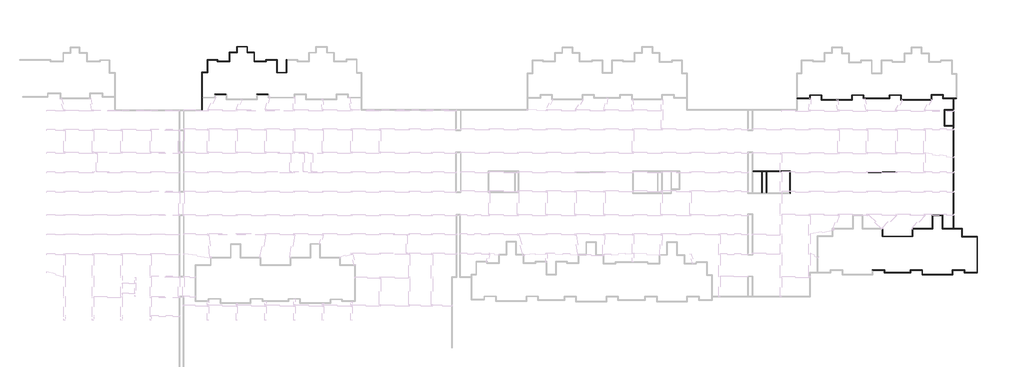
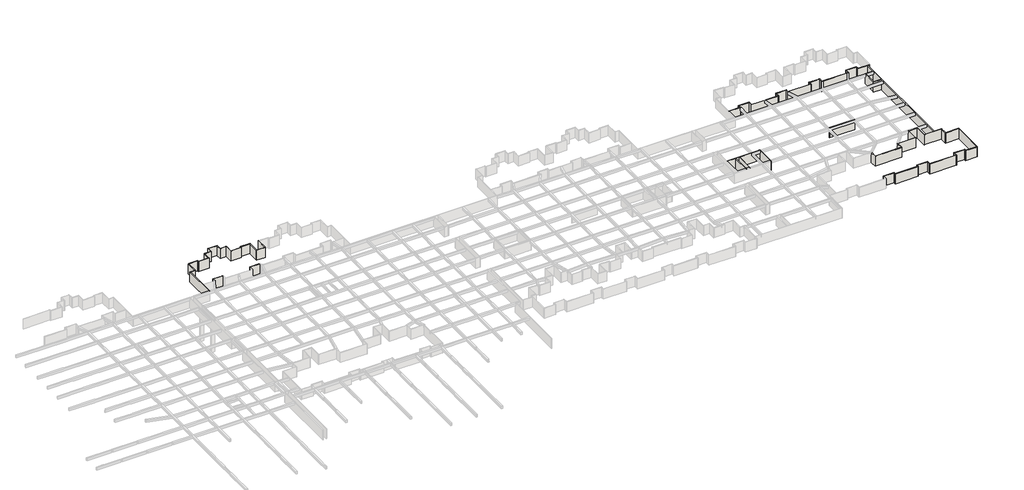
# One storey, part 7 of 16: 69 walls.
"""IFC4 building model written with IfcOpenShell, lengths in millimetres."""

from ifc_helpers import new_model, si_unit, origin, origin_with_axes, place, context, project, spatial, polyline, outline, extrude, faceted_brep, element, save

model = new_model("IFC4")

# Units and contexts
model_context = context("Model", 3, world=origin())
ifc_project = project(units=[si_unit("LENGTHUNIT", "METRE", prefix="MILLI")], contexts=[model_context])

# Site, building, storey
site = spatial("IfcSite", under=ifc_project)
building = spatial("IfcBuilding", under=site)
storey = spatial("IfcBuildingStorey", under=building, Name="户型图", Elevation=0.0)

# Walls
placement = place(None, origin())
element("IfcWall", 1, ObjectType="所有墙体", at=placement, inside=storey, context=model_context, shape_type="Brep", body=[
    faceted_brep([(261322.7517568, -132436.8999905, 0.0), (261322.7517568, -128960.8246701, 0.0), (261322.7517568, -128840.8246701, 0.0), (261322.7517568, -121956.8999905, 0.0), (261322.7517568, -121836.8999905, 0.0), (261322.7517568, -121836.8999905, 3300.0), (261322.7517568, -121956.8999905, 3300.0), (261322.7517568, -128840.8246701, 3300.0), (261322.7517568, -128960.8246701, 3300.0), (261322.7517568, -132436.8999905, 3300.0), (261202.7517568, -132436.8999905, 0.0), (261202.7517568, -132436.8999905, 3300.0), (261202.7517568, -121836.8999905, 3300.0), (261202.7517568, -121836.8999905, 0.0)], [[[0, 1, 2, 3, 4, 5, 6, 7, 8, 9]], [[10, 11, 12, 13]], [[4, 3, 2, 1, 0, 10, 13]], [[9, 8, 7, 6, 5, 12, 11]], [[0, 9, 11, 10]], [[5, 4, 13, 12]]]),
])
element("IfcWall", 2, ObjectType="所有墙体", at=placement, inside=storey, context=model_context, shape_type="Brep", body=[
    faceted_brep([(261322.7517568, -121956.8999905, 0.0), (262826.3863465, -121956.8999905, 0.0), (262826.3863465, -121956.8999905, 3300.0), (261322.7517568, -121956.8999905, 3300.0), (261322.7517568, -121836.8999905, 0.0), (261322.7517568, -121836.8999905, 3300.0), (262706.3863465, -121836.8999905, 3300.0), (262826.3863465, -121836.8999905, 3300.0), (262826.3863465, -121836.8999905, 0.0), (262706.3863465, -121836.8999905, 0.0)], [[[0, 1, 2, 3]], [[4, 5, 6, 7, 8, 9]], [[1, 0, 4, 9, 8]], [[3, 2, 7, 6, 5]], [[0, 3, 5, 4]], [[2, 1, 8, 7]]]),
])
element("IfcWall", 3, ObjectType="所有墙体", at=placement, inside=storey, context=model_context, shape_type="Brep", body=[
    faceted_brep([(262826.3863465, -121836.8999905, 0.0), (262826.3863465, -118414.1462395, 0.0), (262826.3863465, -118294.1462395, 0.0), (262826.3863465, -118294.1462395, 3300.0), (262826.3863465, -118414.1462395, 3300.0), (262826.3863465, -121836.8999905, 3300.0), (262706.3863465, -121836.8999905, 0.0), (262706.3863465, -121836.8999905, 3300.0), (262706.3863465, -118294.1462395, 3300.0), (262706.3863465, -118294.1462395, 0.0)], [[[0, 1, 2, 3, 4, 5]], [[6, 7, 8, 9]], [[2, 1, 0, 6, 9]], [[5, 4, 3, 8, 7]], [[0, 5, 7, 6]], [[3, 2, 9, 8]]]),
])
element("IfcWall", 4, ObjectType="所有墙体", at=placement, inside=storey, context=model_context, shape_type="Brep", body=[
    faceted_brep([(262826.3863465, -118414.1462395, 0.0), (265560.795916, -118414.1462395, 0.0), (265680.795916, -118414.1462395, 0.0), (265680.795916, -118414.1462395, 3300.0), (265560.795916, -118414.1462395, 3300.0), (262826.3863465, -118414.1462395, 3300.0), (262826.3863465, -118294.1462395, 0.0), (262826.3863465, -118294.1462395, 3300.0), (265680.795916, -118294.1462395, 3300.0), (265680.795916, -118294.1462395, 0.0)], [[[0, 1, 2, 3, 4, 5]], [[6, 7, 8, 9]], [[2, 1, 0, 6, 9]], [[5, 4, 3, 8, 7]], [[0, 5, 7, 6]], [[3, 2, 9, 8]]]),
])
element("IfcWall", 5, ObjectType="所有墙体", at=placement, inside=storey, context=model_context, shape_type="Brep", body=[
    faceted_brep([(265560.795916, -118414.1462395, 0.0), (265560.795916, -118816.941108, 0.0), (265560.795916, -118816.941108, 3300.0), (265560.795916, -118414.1462395, 3300.0), (265680.795916, -118414.1462395, 0.0), (265680.795916, -118414.1462395, 3300.0), (265680.795916, -118696.941108, 3300.0), (265680.795916, -118816.941108, 3300.0), (265680.795916, -118816.941108, 0.0), (265680.795916, -118696.941108, 0.0)], [[[0, 1, 2, 3]], [[4, 5, 6, 7, 8, 9]], [[1, 0, 4, 9, 8]], [[3, 2, 7, 6, 5]], [[0, 3, 5, 4]], [[2, 1, 8, 7]]]),
])
element("IfcWall", 6, ObjectType="所有墙体", at=placement, inside=storey, context=model_context, shape_type="Brep", body=[
    faceted_brep([(265680.795916, -118816.941108, 0.0), (268980.795916, -118816.941108, 0.0), (268980.795916, -118816.941108, 3300.0), (265680.795916, -118816.941108, 3300.0), (265680.795916, -118696.941108, 0.0), (265680.795916, -118696.941108, 3300.0), (268860.795916, -118696.941108, 3300.0), (268980.795916, -118696.941108, 3300.0), (268980.795916, -118696.941108, 0.0), (268860.795916, -118696.941108, 0.0)], [[[0, 1, 2, 3]], [[4, 5, 6, 7, 8, 9]], [[1, 0, 4, 9, 8]], [[3, 2, 7, 6, 5]], [[0, 3, 5, 4]], [[2, 1, 8, 7]]]),
])
element("IfcWall", 7, ObjectType="所有墙体", at=placement, inside=storey, context=model_context, shape_type="Brep", body=[
    faceted_brep([(268980.795916, -118696.941108, 0.0), (268980.795916, -116421.0126763, 0.0), (268980.795916, -116301.0126763, 0.0), (268980.795916, -116301.0126763, 3300.0), (268980.795916, -116421.0126763, 3300.0), (268980.795916, -118696.941108, 3300.0), (268860.795916, -118696.941108, 0.0), (268860.795916, -118696.941108, 3300.0), (268860.795916, -116301.0126763, 3300.0), (268860.795916, -116301.0126763, 0.0)], [[[0, 1, 2, 3, 4, 5]], [[6, 7, 8, 9]], [[2, 1, 0, 6, 9]], [[5, 4, 3, 8, 7]], [[0, 5, 7, 6]], [[3, 2, 9, 8]]]),
])
element("IfcWall", 8, ObjectType="所有墙体", at=placement, inside=storey, context=model_context, shape_type="Brep", body=[
    faceted_brep([(268980.795916, -116421.0126763, 0.0), (271083.6374023, -116421.0126763, 0.0), (271083.6374023, -116421.0126763, 3300.0), (268980.795916, -116421.0126763, 3300.0), (268980.795916, -116301.0126763, 0.0), (268980.795916, -116301.0126763, 3300.0), (270963.6374023, -116301.0126763, 3300.0), (271083.6374023, -116301.0126763, 3300.0), (271083.6374023, -116301.0126763, 0.0), (270963.6374023, -116301.0126763, 0.0)], [[[0, 1, 2, 3]], [[4, 5, 6, 7, 8, 9]], [[1, 0, 4, 9, 8]], [[3, 2, 7, 6, 5]], [[0, 3, 5, 4]], [[2, 1, 8, 7]]]),
])
element("IfcWall", 9, ObjectType="所有墙体", at=placement, inside=storey, context=model_context, shape_type="Brep", body=[
    faceted_brep([(271083.6374023, -116301.0126763, 0.0), (271083.6374023, -114773.3023088, 0.0), (271083.6374023, -114653.3023088, 0.0), (271083.6374023, -114653.3023088, 3300.0), (271083.6374023, -114773.3023088, 3300.0), (271083.6374023, -116301.0126763, 3300.0), (270963.6374023, -116301.0126763, 0.0), (270963.6374023, -116301.0126763, 3300.0), (270963.6374023, -114653.3023088, 3300.0), (270963.6374023, -114653.3023088, 0.0)], [[[0, 1, 2, 3, 4, 5]], [[6, 7, 8, 9]], [[2, 1, 0, 6, 9]], [[5, 4, 3, 8, 7]], [[0, 5, 7, 6]], [[3, 2, 9, 8]]]),
])
element("IfcWall", 10, ObjectType="所有墙体", at=placement, inside=storey, context=model_context, shape_type="Brep", body=[
    faceted_brep([(271083.6374023, -114773.3023088, 0.0), (273815.4218707, -114773.3023088, 0.0), (273935.4218707, -114773.3023088, 0.0), (273935.4218707, -114773.3023088, 3300.0), (273815.4218707, -114773.3023088, 3300.0), (271083.6374023, -114773.3023088, 3300.0), (271083.6374023, -114653.3023088, 0.0), (271083.6374023, -114653.3023088, 3300.0), (273935.4218707, -114653.3023088, 3300.0), (273935.4218707, -114653.3023088, 0.0)], [[[0, 1, 2, 3, 4, 5]], [[6, 7, 8, 9]], [[2, 1, 0, 6, 9]], [[5, 4, 3, 8, 7]], [[0, 5, 7, 6]], [[3, 2, 9, 8]]]),
])
element("IfcWall", 11, ObjectType="所有墙体", at=placement, inside=storey, context=model_context, shape_type="Brep", body=[
    faceted_brep([(273815.4218707, -114773.3023088, 0.0), (273815.4218707, -116421.0126763, 0.0), (273815.4218707, -116421.0126763, 3300.0), (273815.4218707, -114773.3023088, 3300.0), (273935.4218707, -114773.3023088, 0.0), (273935.4218707, -114773.3023088, 3300.0), (273935.4218707, -116301.0126763, 3300.0), (273935.4218707, -116421.0126763, 3300.0), (273935.4218707, -116421.0126763, 0.0), (273935.4218707, -116301.0126763, 0.0)], [[[0, 1, 2, 3]], [[4, 5, 6, 7, 8, 9]], [[1, 0, 4, 9, 8]], [[3, 2, 7, 6, 5]], [[0, 3, 5, 4]], [[2, 1, 8, 7]]]),
])
element("IfcWall", 12, ObjectType="所有墙体", at=placement, inside=storey, context=model_context, shape_type="Brep", body=[
    faceted_brep([(273935.4218707, -116421.0126763, 0.0), (275763.6122444, -116421.0126763, 0.0), (275883.6122444, -116421.0126763, 0.0), (275883.6122444, -116421.0126763, 3300.0), (275763.6122444, -116421.0126763, 3300.0), (273935.4218707, -116421.0126763, 3300.0), (273935.4218707, -116301.0126763, 0.0), (273935.4218707, -116301.0126763, 3300.0), (275883.6122444, -116301.0126763, 3300.0), (275883.6122444, -116301.0126763, 0.0)], [[[0, 1, 2, 3, 4, 5]], [[6, 7, 8, 9]], [[2, 1, 0, 6, 9]], [[5, 4, 3, 8, 7]], [[0, 5, 7, 6]], [[3, 2, 9, 8]]]),
])
element("IfcWall", 13, ObjectType="所有墙体", at=placement, inside=storey, context=model_context, shape_type="Brep", body=[
    faceted_brep([(275763.6122444, -116421.0126763, 0.0), (275763.6122444, -118816.941108, 0.0), (275763.6122444, -118816.941108, 3300.0), (275763.6122444, -116421.0126763, 3300.0), (275883.6122444, -116421.0126763, 0.0), (275883.6122444, -116421.0126763, 3300.0), (275883.6122444, -118696.941108, 3300.0), (275883.6122444, -118816.941108, 3300.0), (275883.6122444, -118816.941108, 0.0), (275883.6122444, -118696.941108, 0.0)], [[[0, 1, 2, 3]], [[4, 5, 6, 7, 8, 9]], [[1, 0, 4, 9, 8]], [[3, 2, 7, 6, 5]], [[0, 3, 5, 4]], [[2, 1, 8, 7]]]),
])
element("IfcWall", 14, ObjectType="所有墙体", at=placement, inside=storey, context=model_context, shape_type="Brep", body=[
    faceted_brep([(275883.6122444, -118816.941108, 0.0), (279180.1877082, -118816.941108, 0.0), (279180.1877082, -118816.941108, 3300.0), (275883.6122444, -118816.941108, 3300.0), (275883.6122444, -118696.941108, 0.0), (275883.6122444, -118696.941108, 3300.0), (279060.1877082, -118696.941108, 3300.0), (279180.1877082, -118696.941108, 3300.0), (279180.1877082, -118696.941108, 0.0), (279060.1877082, -118696.941108, 0.0)], [[[0, 1, 2, 3]], [[4, 5, 6, 7, 8, 9]], [[1, 0, 4, 9, 8]], [[3, 2, 7, 6, 5]], [[0, 3, 5, 4]], [[2, 1, 8, 7]]]),
])
element("IfcWall", 15, ObjectType="所有墙体", at=placement, inside=storey, context=model_context, shape_type="Brep", body=[
    faceted_brep([(279180.1877082, -118696.941108, 0.0), (279180.1877082, -118416.941108, 0.0), (279180.1877082, -118296.941108, 0.0), (279180.1877082, -118296.941108, 3300.0), (279180.1877082, -118416.941108, 3300.0), (279180.1877082, -118696.941108, 3300.0), (279060.1877082, -118696.941108, 0.0), (279060.1877082, -118696.941108, 3300.0), (279060.1877082, -118296.941108, 3300.0), (279060.1877082, -118296.941108, 0.0)], [[[0, 1, 2, 3, 4, 5]], [[6, 7, 8, 9]], [[2, 1, 0, 6, 9]], [[5, 4, 3, 8, 7]], [[0, 5, 7, 6]], [[3, 2, 9, 8]]]),
])
element("IfcWall", 16, ObjectType="所有墙体", at=placement, inside=storey, context=model_context, shape_type="Brep", body=[
    faceted_brep([(279180.1877082, -118416.941108, 0.0), (282060.1877082, -118416.941108, 0.0), (282180.1877082, -118416.941108, 0.0), (282180.1877082, -118416.941108, 3300.0), (282060.1877082, -118416.941108, 3300.0), (279180.1877082, -118416.941108, 3300.0), (279180.1877082, -118296.941108, 0.0), (279180.1877082, -118296.941108, 3300.0), (282180.1877082, -118296.941108, 3300.0), (282180.1877082, -118296.941108, 0.0)], [[[0, 1, 2, 3, 4, 5]], [[6, 7, 8, 9]], [[2, 1, 0, 6, 9]], [[5, 4, 3, 8, 7]], [[0, 5, 7, 6]], [[3, 2, 9, 8]]]),
])
element("IfcWall", 17, ObjectType="所有墙体", at=placement, inside=storey, context=model_context, shape_type="Brep", body=[
    faceted_brep([(282060.1877082, -118416.941108, 0.0), (282060.1877082, -122016.941108, 0.0), (282060.1877082, -122016.941108, 3300.0), (282060.1877082, -118416.941108, 3300.0), (282180.1877082, -118416.941108, 0.0), (282180.1877082, -118416.941108, 3300.0), (282180.1877082, -121896.941108, 3300.0), (282180.1877082, -122016.941108, 3300.0), (282180.1877082, -122016.941108, 0.0), (282180.1877082, -121896.941108, 0.0)], [[[0, 1, 2, 3]], [[4, 5, 6, 7, 8, 9]], [[1, 0, 4, 9, 8]], [[3, 2, 7, 6, 5]], [[0, 3, 5, 4]], [[2, 1, 8, 7]]]),
])
element("IfcWall", 18, ObjectType="所有墙体", at=placement, inside=storey, context=model_context, shape_type="Brep", body=[
    faceted_brep([(282180.1877082, -122016.941108, 0.0), (284876.4528769, -122016.941108, 0.0), (284876.4528769, -122016.941108, 3300.0), (282180.1877082, -122016.941108, 3300.0), (282180.1877082, -121896.941108, 0.0), (282180.1877082, -121896.941108, 3300.0), (284756.4528769, -121896.941108, 3300.0), (284876.4528769, -121896.941108, 3300.0), (284876.4528769, -121896.941108, 0.0), (284756.4528769, -121896.941108, 0.0)], [[[0, 1, 2, 3]], [[4, 5, 6, 7, 8, 9]], [[1, 0, 4, 9, 8]], [[3, 2, 7, 6, 5]], [[0, 3, 5, 4]], [[2, 1, 8, 7]]]),
])
element("IfcWall", 19, ObjectType="所有墙体", at=placement, inside=storey, context=model_context, shape_type="Brep", body=[
    faceted_brep([(284876.4528769, -121896.941108, 0.0), (284876.4528769, -118416.941108, 0.0), (284876.4528769, -118296.941108, 0.0), (284876.4528769, -118296.941108, 3300.0), (284876.4528769, -118416.941108, 3300.0), (284876.4528769, -121896.941108, 3300.0), (284756.4528769, -121896.941108, 0.0), (284756.4528769, -121896.941108, 3300.0), (284756.4528769, -118296.941108, 3300.0), (284756.4528769, -118296.941108, 0.0)], [[[0, 1, 2, 3, 4, 5]], [[6, 7, 8, 9]], [[2, 1, 0, 6, 9]], [[5, 4, 3, 8, 7]], [[0, 5, 7, 6]], [[3, 2, 9, 8]]]),
])
element("IfcWall", 20, ObjectType="所有墙体", at=placement, inside=storey, context=model_context, shape_type="Brep", body=[
    faceted_brep([(279699.0680425, -127937.9986276, 0.0), (276499.7065412, -127937.9986276, 0.0), (276499.7065412, -127937.9986276, 3300.0), (279699.0680425, -127937.9986276, 3300.0), (279699.0680425, -128057.9986276, 0.0), (279699.0680425, -128057.9986276, 3300.0), (276619.7065412, -128057.9986276, 3300.0), (276499.7065412, -128057.9986276, 3300.0), (276499.7065412, -128057.9986276, 0.0), (276619.7065412, -128057.9986276, 0.0)], [[[0, 1, 2, 3]], [[4, 5, 6, 7, 8, 9]], [[1, 0, 4, 9, 8]], [[3, 2, 7, 6, 5]], [[0, 3, 5, 4]], [[2, 1, 8, 7]]]),
])
element("IfcWall", 21, ObjectType="所有墙体", at=placement, inside=storey, context=model_context, shape_type="Brep", body=[
    faceted_brep([(267998.1706199, -127937.9986276, 0.0), (264899.6993188, -127937.9986276, 0.0), (264899.6993188, -127937.9986276, 3300.0), (267998.1706199, -127937.9986276, 3300.0), (267998.1706199, -128057.9986276, 0.0), (267998.1706199, -128057.9986276, 3300.0), (265019.6993188, -128057.9986276, 3300.0), (264899.6993188, -128057.9986276, 3300.0), (264899.6993188, -128057.9986276, 0.0), (265019.6993188, -128057.9986276, 0.0)], [[[0, 1, 2, 3]], [[4, 5, 6, 7, 8, 9]], [[1, 0, 4, 9, 8]], [[3, 2, 7, 6, 5]], [[0, 3, 5, 4]], [[2, 1, 8, 7]]]),
])
element("IfcWall", 22, ObjectType="所有墙体", at=placement, inside=storey, context=model_context, shape_type="Brep", body=[
    faceted_brep([(471205.459909, -129026.8599361, 0.0), (467617.8679483, -129026.8599361, 0.0), (467497.8679483, -129026.8599361, 0.0), (467497.8679483, -129026.8599361, 3300.0), (467617.8679483, -129026.8599361, 3300.0), (471205.459909, -129026.8599361, 3300.0), (471205.459909, -129146.8599361, 0.0), (471205.459909, -129146.8599361, 3300.0), (470565.459909, -129146.8599361, 3300.0), (470445.459909, -129146.8599361, 3300.0), (467497.8679483, -129146.8599361, 3300.0), (467497.8679483, -129146.8599361, 0.0), (470445.459909, -129146.8599361, 0.0), (470565.459909, -129146.8599361, 0.0)], [[[0, 1, 2, 3, 4, 5]], [[6, 7, 8, 9, 10, 11, 12, 13]], [[2, 1, 0, 6, 13, 12, 11]], [[5, 4, 3, 10, 9, 8, 7]], [[0, 5, 7, 6]], [[3, 2, 11, 10]]]),
])
element("IfcWall", 23, ObjectType="所有墙体", at=placement, inside=storey, context=model_context, shape_type="Brep", body=[
    faceted_brep([(467617.8679483, -129026.8599361, 0.0), (467617.8679483, -128122.7220843, 0.0), (467617.8679483, -128122.7220843, 3300.0), (467617.8679483, -129026.8599361, 3300.0), (467497.8679483, -129026.8599361, 0.0), (467497.8679483, -129026.8599361, 3300.0), (467497.8679483, -128242.7220843, 3300.0), (467497.8679483, -128122.7220843, 3300.0), (467497.8679483, -128122.7220843, 0.0), (467497.8679483, -128242.7220843, 0.0)], [[[0, 1, 2, 3]], [[4, 5, 6, 7, 8, 9]], [[1, 0, 4, 9, 8]], [[3, 2, 7, 6, 5]], [[0, 3, 5, 4]], [[2, 1, 8, 7]]]),
])
element("IfcWall", 24, ObjectType="所有墙体", at=placement, inside=storey, context=model_context, shape_type="Brep", body=[
    faceted_brep([(467497.8679483, -128122.7220843, 0.0), (464298.8748808, -128122.7220843, 0.0), (464298.8748808, -128122.7220843, 3300.0), (467497.8679483, -128122.7220843, 3300.0), (467497.8679483, -128242.7220843, 0.0), (467497.8679483, -128242.7220843, 3300.0), (464418.8748808, -128242.7220843, 3300.0), (464298.8748808, -128242.7220843, 3300.0), (464298.8748808, -128242.7220843, 0.0), (464418.8748808, -128242.7220843, 0.0)], [[[0, 1, 2, 3]], [[4, 5, 6, 7, 8, 9]], [[1, 0, 4, 9, 8]], [[3, 2, 7, 6, 5]], [[0, 3, 5, 4]], [[2, 1, 8, 7]]]),
])
element("IfcWall", 25, ObjectType="所有墙体", at=placement, inside=storey, context=model_context, shape_type="Brep", body=[
    faceted_brep([(464298.8748808, -128242.7220843, 0.0), (464298.8748808, -129422.7220843, 0.0), (464298.8748808, -129542.7220843, 0.0), (464298.8748808, -129542.7220843, 3300.0), (464298.8748808, -129422.7220843, 3300.0), (464298.8748808, -128242.7220843, 3300.0), (464418.8748808, -128242.7220843, 0.0), (464418.8748808, -128242.7220843, 3300.0), (464418.8748808, -129542.7220843, 3300.0), (464418.8748808, -129542.7220843, 0.0)], [[[0, 1, 2, 3, 4, 5]], [[6, 7, 8, 9]], [[2, 1, 0, 6, 9]], [[5, 4, 3, 8, 7]], [[0, 5, 7, 6]], [[3, 2, 9, 8]]]),
])
element("IfcWall", 26, ObjectType="所有墙体", at=placement, inside=storey, context=model_context, shape_type="Brep", body=[
    faceted_brep([(464298.8748808, -129422.7220843, 0.0), (455978.8748808, -129422.7220843, 0.0), (455858.8748808, -129422.7220843, 0.0), (455858.8748808, -129422.7220843, 3300.0), (455978.8748808, -129422.7220843, 3300.0), (464298.8748808, -129422.7220843, 3300.0), (464298.8748808, -129542.7220843, 0.0), (464298.8748808, -129542.7220843, 3300.0), (455858.8748808, -129542.7220843, 3300.0), (455858.8748808, -129542.7220843, 0.0)], [[[0, 1, 2, 3, 4, 5]], [[6, 7, 8, 9]], [[2, 1, 0, 6, 9]], [[5, 4, 3, 8, 7]], [[0, 5, 7, 6]], [[3, 2, 9, 8]]]),
])
element("IfcWall", 27, ObjectType="所有墙体", at=placement, inside=storey, context=model_context, shape_type="Brep", body=[
    faceted_brep([(455978.8748808, -129422.7220843, 0.0), (455978.8748808, -128142.7220843, 0.0), (455978.8748808, -128142.7220843, 3300.0), (455978.8748808, -129422.7220843, 3300.0), (455858.8748808, -129422.7220843, 0.0), (455858.8748808, -129422.7220843, 3300.0), (455858.8748808, -128262.7220843, 3300.0), (455858.8748808, -128142.7220843, 3300.0), (455858.8748808, -128142.7220843, 0.0), (455858.8748808, -128262.7220843, 0.0)], [[[0, 1, 2, 3]], [[4, 5, 6, 7, 8, 9]], [[1, 0, 4, 9, 8]], [[3, 2, 7, 6, 5]], [[0, 3, 5, 4]], [[2, 1, 8, 7]]]),
])
element("IfcWall", 28, ObjectType="所有墙体", at=placement, inside=storey, context=model_context, shape_type="Brep", body=[
    faceted_brep([(455858.8748808, -128142.7220843, 0.0), (452638.8748808, -128142.7220843, 0.0), (452638.8748808, -128142.7220843, 3300.0), (455858.8748808, -128142.7220843, 3300.0), (455858.8748808, -128262.7220843, 0.0), (455858.8748808, -128262.7220843, 3300.0), (452758.8748808, -128262.7220843, 3300.0), (452638.8748808, -128262.7220843, 3300.0), (452638.8748808, -128262.7220843, 0.0), (452758.8748808, -128262.7220843, 0.0)], [[[0, 1, 2, 3]], [[4, 5, 6, 7, 8, 9]], [[1, 0, 4, 9, 8]], [[3, 2, 7, 6, 5]], [[0, 3, 5, 4]], [[2, 1, 8, 7]]]),
])
element("IfcWall", 29, ObjectType="所有墙体", at=placement, inside=storey, context=model_context, shape_type="Brep", body=[
    faceted_brep([(452638.8748808, -128262.7220843, 0.0), (452638.8748808, -129042.7220843, 0.0), (452638.8748808, -129162.7220843, 0.0), (452638.8748808, -129162.7220843, 3300.0), (452638.8748808, -129042.7220843, 3300.0), (452638.8748808, -128262.7220843, 3300.0), (452758.8748808, -128262.7220843, 0.0), (452758.8748808, -128262.7220843, 3300.0), (452758.8748808, -129162.7220843, 3300.0), (452758.8748808, -129162.7220843, 0.0)], [[[0, 1, 2, 3, 4, 5]], [[6, 7, 8, 9]], [[2, 1, 0, 6, 9]], [[5, 4, 3, 8, 7]], [[0, 5, 7, 6]], [[3, 2, 9, 8]]]),
])
element("IfcWall", 30, ObjectType="所有墙体", at=placement, inside=storey, context=model_context, shape_type="Brep", body=[
    faceted_brep([(452638.8748808, -129042.7220843, 0.0), (445498.8748808, -129042.7220843, 0.0), (445378.8748808, -129042.7220843, 0.0), (445378.8748808, -129042.7220843, 3300.0), (445498.8748808, -129042.7220843, 3300.0), (452638.8748808, -129042.7220843, 3300.0), (452638.8748808, -129162.7220843, 0.0), (452638.8748808, -129162.7220843, 3300.0), (445378.8748808, -129162.7220843, 3300.0), (445378.8748808, -129162.7220843, 0.0)], [[[0, 1, 2, 3, 4, 5]], [[6, 7, 8, 9]], [[2, 1, 0, 6, 9]], [[5, 4, 3, 8, 7]], [[0, 5, 7, 6]], [[3, 2, 9, 8]]]),
])
element("IfcWall", 31, ObjectType="所有墙体", at=placement, inside=storey, context=model_context, shape_type="Brep", body=[
    faceted_brep([(445498.8748808, -129042.7220843, 0.0), (445498.8748808, -128142.7220843, 0.0), (445498.8748808, -128142.7220843, 3300.0), (445498.8748808, -129042.7220843, 3300.0), (445378.8748808, -129042.7220843, 0.0), (445378.8748808, -129042.7220843, 3300.0), (445378.8748808, -128262.7220843, 3300.0), (445378.8748808, -128142.7220843, 3300.0), (445378.8748808, -128142.7220843, 0.0), (445378.8748808, -128262.7220843, 0.0)], [[[0, 1, 2, 3]], [[4, 5, 6, 7, 8, 9]], [[1, 0, 4, 9, 8]], [[3, 2, 7, 6, 5]], [[0, 3, 5, 4]], [[2, 1, 8, 7]]]),
])
element("IfcWall", 32, ObjectType="所有墙体", at=placement, inside=storey, context=model_context, shape_type="Brep", body=[
    faceted_brep([(445378.8748808, -128142.7220843, 0.0), (442158.8748808, -128142.7220843, 0.0), (442158.8748808, -128142.7220843, 3300.0), (445378.8748808, -128142.7220843, 3300.0), (445378.8748808, -128262.7220843, 0.0), (445378.8748808, -128262.7220843, 3300.0), (442278.8748808, -128262.7220843, 3300.0), (442158.8748808, -128262.7220843, 3300.0), (442158.8748808, -128262.7220843, 0.0), (442278.8748808, -128262.7220843, 0.0)], [[[0, 1, 2, 3]], [[4, 5, 6, 7, 8, 9]], [[1, 0, 4, 9, 8]], [[3, 2, 7, 6, 5]], [[0, 3, 5, 4]], [[2, 1, 8, 7]]]),
])
element("IfcWall", 33, ObjectType="所有墙体", at=placement, inside=storey, context=model_context, shape_type="Brep", body=[
    faceted_brep([(442158.8748808, -128262.7220843, 0.0), (442158.8748808, -129422.7220843, 0.0), (442158.8748808, -129542.7220843, 0.0), (442158.8748808, -129542.7220843, 3300.0), (442158.8748808, -129422.7220843, 3300.0), (442158.8748808, -128262.7220843, 3300.0), (442278.8748808, -128262.7220843, 0.0), (442278.8748808, -128262.7220843, 3300.0), (442278.8748808, -129542.7220843, 3300.0), (442278.8748808, -129542.7220843, 0.0)], [[[0, 1, 2, 3, 4, 5]], [[6, 7, 8, 9]], [[2, 1, 0, 6, 9]], [[5, 4, 3, 8, 7]], [[0, 5, 7, 6]], [[3, 2, 9, 8]]]),
])
element("IfcWall", 34, ObjectType="所有墙体", at=placement, inside=storey, context=model_context, shape_type="Brep", body=[
    faceted_brep([(442158.8748808, -129422.7220843, 0.0), (433817.4051625, -129422.7220843, 0.0), (433697.4051625, -129422.7220843, 0.0), (433697.4051625, -129422.7220843, 3300.0), (433817.4051625, -129422.7220843, 3300.0), (442158.8748808, -129422.7220843, 3300.0), (442158.8748808, -129542.7220843, 0.0), (442158.8748808, -129542.7220843, 3300.0), (433697.4051625, -129542.7220843, 3300.0), (433697.4051625, -129542.7220843, 0.0)], [[[0, 1, 2, 3, 4, 5]], [[6, 7, 8, 9]], [[2, 1, 0, 6, 9]], [[5, 4, 3, 8, 7]], [[0, 5, 7, 6]], [[3, 2, 9, 8]]]),
])
element("IfcWall", 35, ObjectType="所有墙体", at=placement, inside=storey, context=model_context, shape_type="Brep", body=[
    faceted_brep([(433817.4051625, -129422.7220843, 0.0), (433817.4051625, -128142.7220843, 0.0), (433817.4051625, -128142.7220843, 3300.0), (433817.4051625, -129422.7220843, 3300.0), (433697.4051625, -129422.7220843, 0.0), (433697.4051625, -129422.7220843, 3300.0), (433697.4051625, -128262.7220843, 3300.0), (433697.4051625, -128142.7220843, 3300.0), (433697.4051625, -128142.7220843, 0.0), (433697.4051625, -128262.7220843, 0.0)], [[[0, 1, 2, 3]], [[4, 5, 6, 7, 8, 9]], [[1, 0, 4, 9, 8]], [[3, 2, 7, 6, 5]], [[0, 3, 5, 4]], [[2, 1, 8, 7]]]),
])
element("IfcWall", 36, ObjectType="所有墙体", at=placement, inside=storey, context=model_context, shape_type="Brep", body=[
    faceted_brep([(433697.4051625, -128142.7220843, 0.0), (430445.4085156, -128142.7220843, 0.0), (430445.4085156, -128142.7220843, 3300.0), (433697.4051625, -128142.7220843, 3300.0), (433697.4051625, -128262.7220843, 0.0), (433697.4051625, -128262.7220843, 3300.0), (430565.4085156, -128262.7220843, 3300.0), (430445.4085156, -128262.7220843, 3300.0), (430445.4085156, -128262.7220843, 0.0), (430565.4085156, -128262.7220843, 0.0)], [[[0, 1, 2, 3]], [[4, 5, 6, 7, 8, 9]], [[1, 0, 4, 9, 8]], [[3, 2, 7, 6, 5]], [[0, 3, 5, 4]], [[2, 1, 8, 7]]]),
])
element("IfcWall", 37, ObjectType="所有墙体", at=placement, inside=storey, context=model_context, shape_type="Brep", body=[
    faceted_brep([(430445.4085156, -128262.7220843, 0.0), (430445.4085156, -129042.7220843, 0.0), (430445.4085156, -129162.7220843, 0.0), (430445.4085156, -129162.7220843, 3300.0), (430445.4085156, -129042.7220843, 3300.0), (430445.4085156, -128262.7220843, 3300.0), (430565.4085156, -128262.7220843, 0.0), (430565.4085156, -128262.7220843, 3300.0), (430565.4085156, -129162.7220843, 3300.0), (430565.4085156, -129162.7220843, 0.0)], [[[0, 1, 2, 3, 4, 5]], [[6, 7, 8, 9]], [[2, 1, 0, 6, 9]], [[5, 4, 3, 8, 7]], [[0, 5, 7, 6]], [[3, 2, 9, 8]]]),
])
element("IfcWall", 38, ObjectType="所有墙体", at=placement, inside=storey, context=model_context, shape_type="SweptSolid", body=[
    extrude(outline(polyline([(426925.7298502, -129042.7220843), (430445.4085156, -129042.7220843), (430445.4085156, -129162.7220843), (426925.7298502, -129162.7220843), (426925.7298502, -129042.7220843)])), origin_with_axes(), (0.0, 0.0, 1.0), 3300.0),
])
element("IfcWall", 39, ObjectType="所有墙体", at=placement, inside=storey, context=model_context, shape_type="Brep", body=[
    faceted_brep([(470445.459909, -129146.8599361, 0.0), (470445.459909, -132245.1471774, 0.0), (470445.459909, -132365.1471774, 0.0), (470445.459909, -136745.1471774, 0.0), (470445.459909, -136865.1471774, 0.0), (470445.459909, -165426.8599361, 0.0), (470445.459909, -165426.8599361, 3300.0), (470445.459909, -136865.1471774, 3300.0), (470445.459909, -136745.1471774, 3300.0), (470445.459909, -132365.1471774, 3300.0), (470445.459909, -132245.1471774, 3300.0), (470445.459909, -129146.8599361, 3300.0), (470565.459909, -129146.8599361, 0.0), (470565.459909, -129146.8599361, 3300.0), (470565.459909, -165426.8599361, 3300.0), (470565.459909, -165426.8599361, 0.0)], [[[0, 1, 2, 3, 4, 5, 6, 7, 8, 9, 10, 11]], [[12, 13, 14, 15]], [[5, 4, 3, 2, 1, 0, 12, 15]], [[11, 10, 9, 8, 7, 6, 14, 13]], [[0, 11, 13, 12]], [[6, 5, 15, 14]]]),
])
element("IfcWall", 40, ObjectType="所有墙体", at=placement, inside=storey, context=model_context, shape_type="Brep", body=[
    faceted_brep([(467447.0448848, -165546.8599361, 0.0), (472821.8487608, -165546.8599361, 0.0), (472941.8487608, -165546.8599361, 0.0), (472941.8487608, -165546.8599361, 3300.0), (472821.8487608, -165546.8599361, 3300.0), (467447.0448848, -165546.8599361, 3300.0), (467447.0448848, -165426.8599361, 0.0), (467447.0448848, -165426.8599361, 3300.0), (470445.459909, -165426.8599361, 3300.0), (470565.459909, -165426.8599361, 3300.0), (472941.8487608, -165426.8599361, 3300.0), (472941.8487608, -165426.8599361, 0.0), (470565.459909, -165426.8599361, 0.0), (470445.459909, -165426.8599361, 0.0)], [[[0, 1, 2, 3, 4, 5]], [[6, 7, 8, 9, 10, 11, 12, 13]], [[2, 1, 0, 6, 13, 12, 11]], [[5, 4, 3, 10, 9, 8, 7]], [[3, 2, 11, 10]], [[0, 5, 7, 6]]]),
])
element("IfcWall", 41, ObjectType="所有墙体", at=placement, inside=storey, context=model_context, shape_type="Brep", body=[
    faceted_brep([(472821.8487608, -165546.8599361, 0.0), (472821.8487608, -167696.2427987, 0.0), (472821.8487608, -167696.2427987, 3300.0), (472821.8487608, -165546.8599361, 3300.0), (472941.8487608, -165546.8599361, 0.0), (472941.8487608, -165546.8599361, 3300.0), (472941.8487608, -167576.2427987, 3300.0), (472941.8487608, -167696.2427987, 3300.0), (472941.8487608, -167696.2427987, 0.0), (472941.8487608, -167576.2427987, 0.0)], [[[0, 1, 2, 3]], [[4, 5, 6, 7, 8, 9]], [[1, 0, 4, 9, 8]], [[3, 2, 7, 6, 5]], [[0, 3, 5, 4]], [[2, 1, 8, 7]]]),
])
element("IfcWall", 42, ObjectType="所有墙体", at=placement, inside=storey, context=model_context, shape_type="Brep", body=[
    faceted_brep([(472941.8487608, -167696.2427987, 0.0), (477020.7360443, -167696.2427987, 0.0), (477140.7360443, -167696.2427987, 0.0), (477140.7360443, -167696.2427987, 3300.0), (477020.7360443, -167696.2427987, 3300.0), (472941.8487608, -167696.2427987, 3300.0), (472941.8487608, -167576.2427987, 0.0), (472941.8487608, -167576.2427987, 3300.0), (477140.7360443, -167576.2427987, 3300.0), (477140.7360443, -167576.2427987, 0.0)], [[[0, 1, 2, 3, 4, 5]], [[6, 7, 8, 9]], [[2, 1, 0, 6, 9]], [[5, 4, 3, 8, 7]], [[0, 5, 7, 6]], [[3, 2, 9, 8]]]),
])
element("IfcWall", 43, ObjectType="所有墙体", at=placement, inside=storey, context=model_context, shape_type="Brep", body=[
    faceted_brep([(477020.7360443, -167696.2427987, 0.0), (477020.7360443, -177576.2427987, 0.0), (477020.7360443, -177696.2427987, 0.0), (477020.7360443, -177696.2427987, 3300.0), (477020.7360443, -177576.2427987, 3300.0), (477020.7360443, -167696.2427987, 3300.0), (477140.7360443, -167696.2427987, 0.0), (477140.7360443, -167696.2427987, 3300.0), (477140.7360443, -177696.2427987, 3300.0), (477140.7360443, -177696.2427987, 0.0)], [[[0, 1, 2, 3, 4, 5]], [[6, 7, 8, 9]], [[2, 1, 0, 6, 9]], [[5, 4, 3, 8, 7]], [[0, 5, 7, 6]], [[3, 2, 9, 8]]]),
])
element("IfcWall", 44, ObjectType="所有墙体", at=placement, inside=storey, context=model_context, shape_type="Brep", body=[
    faceted_brep([(477020.7360443, -177576.2427987, 0.0), (473540.7360443, -177576.2427987, 0.0), (473420.7360443, -177576.2427987, 0.0), (473420.7360443, -177576.2427987, 3300.0), (473540.7360443, -177576.2427987, 3300.0), (477020.7360443, -177576.2427987, 3300.0), (477020.7360443, -177696.2427987, 0.0), (477020.7360443, -177696.2427987, 3300.0), (473420.7360443, -177696.2427987, 3300.0), (473420.7360443, -177696.2427987, 0.0)], [[[0, 1, 2, 3, 4, 5]], [[6, 7, 8, 9]], [[2, 1, 0, 6, 9]], [[5, 4, 3, 8, 7]], [[0, 5, 7, 6]], [[3, 2, 9, 8]]]),
])
element("IfcWall", 45, ObjectType="所有墙体", at=placement, inside=storey, context=model_context, shape_type="Brep", body=[
    faceted_brep([(473540.7360443, -177576.2427987, 0.0), (473540.7360443, -176976.9317024, 0.0), (473540.7360443, -176976.9317024, 3300.0), (473540.7360443, -177576.2427987, 3300.0), (473420.7360443, -177576.2427987, 0.0), (473420.7360443, -177576.2427987, 3300.0), (473420.7360443, -177096.9317024, 3300.0), (473420.7360443, -176976.9317024, 3300.0), (473420.7360443, -176976.9317024, 0.0), (473420.7360443, -177096.9317024, 0.0)], [[[0, 1, 2, 3]], [[4, 5, 6, 7, 8, 9]], [[1, 0, 4, 9, 8]], [[3, 2, 7, 6, 5]], [[0, 3, 5, 4]], [[2, 1, 8, 7]]]),
])
element("IfcWall", 46, ObjectType="所有墙体", at=placement, inside=storey, context=model_context, shape_type="Brep", body=[
    faceted_brep([(473420.7360443, -176976.9317024, 0.0), (470110.2415677, -176976.9317024, 0.0), (470110.2415677, -176976.9317024, 3300.0), (473420.7360443, -176976.9317024, 3300.0), (473420.7360443, -177096.9317024, 0.0), (473420.7360443, -177096.9317024, 3300.0), (470230.2415677, -177096.9317024, 3300.0), (470110.2415677, -177096.9317024, 3300.0), (470110.2415677, -177096.9317024, 0.0), (470230.2415677, -177096.9317024, 0.0)], [[[0, 1, 2, 3]], [[4, 5, 6, 7, 8, 9]], [[1, 0, 4, 9, 8]], [[3, 2, 7, 6, 5]], [[0, 3, 5, 4]], [[2, 1, 8, 7]]]),
])
element("IfcWall", 47, ObjectType="所有墙体", at=placement, inside=storey, context=model_context, shape_type="Brep", body=[
    faceted_brep([(470110.2415677, -177096.9317024, 0.0), (470110.2415677, -178176.9317024, 0.0), (470110.2415677, -178296.9317024, 0.0), (470110.2415677, -178296.9317024, 3300.0), (470110.2415677, -178176.9317024, 3300.0), (470110.2415677, -177096.9317024, 3300.0), (470230.2415677, -177096.9317024, 0.0), (470230.2415677, -177096.9317024, 3300.0), (470230.2415677, -178296.9317024, 3300.0), (470230.2415677, -178296.9317024, 0.0)], [[[0, 1, 2, 3, 4, 5]], [[6, 7, 8, 9]], [[2, 1, 0, 6, 9]], [[5, 4, 3, 8, 7]], [[0, 5, 7, 6]], [[3, 2, 9, 8]]]),
])
element("IfcWall", 48, ObjectType="所有墙体", at=placement, inside=storey, context=model_context, shape_type="Brep", body=[
    faceted_brep([(470110.2415677, -178176.9317024, 0.0), (461828.8953338, -178176.9317024, 0.0), (461708.8953338, -178176.9317024, 0.0), (461708.8953338, -178176.9317024, 3300.0), (461828.8953338, -178176.9317024, 3300.0), (470110.2415677, -178176.9317024, 3300.0), (470110.2415677, -178296.9317024, 0.0), (470110.2415677, -178296.9317024, 3300.0), (461708.8953338, -178296.9317024, 3300.0), (461708.8953338, -178296.9317024, 0.0)], [[[0, 1, 2, 3, 4, 5]], [[6, 7, 8, 9]], [[2, 1, 0, 6, 9]], [[5, 4, 3, 8, 7]], [[0, 5, 7, 6]], [[3, 2, 9, 8]]]),
])
element("IfcWall", 49, ObjectType="所有墙体", at=placement, inside=storey, context=model_context, shape_type="Brep", body=[
    faceted_brep([(461828.8953338, -178176.9317024, 0.0), (461828.8953338, -176976.9317024, 0.0), (461828.8953338, -176976.9317024, 3300.0), (461828.8953338, -178176.9317024, 3300.0), (461708.8953338, -178176.9317024, 0.0), (461708.8953338, -178176.9317024, 3300.0), (461708.8953338, -177096.9317024, 3300.0), (461708.8953338, -176976.9317024, 3300.0), (461708.8953338, -176976.9317024, 0.0), (461708.8953338, -177096.9317024, 0.0)], [[[0, 1, 2, 3]], [[4, 5, 6, 7, 8, 9]], [[1, 0, 4, 9, 8]], [[3, 2, 7, 6, 5]], [[0, 3, 5, 4]], [[2, 1, 8, 7]]]),
])
element("IfcWall", 50, ObjectType="所有墙体", at=placement, inside=storey, context=model_context, shape_type="Brep", body=[
    faceted_brep([(461708.8953338, -176976.9317024, 0.0), (458408.8953338, -176976.9317024, 0.0), (458408.8953338, -176976.9317024, 3300.0), (461708.8953338, -176976.9317024, 3300.0), (461708.8953338, -177096.9317024, 0.0), (461708.8953338, -177096.9317024, 3300.0), (458528.8953338, -177096.9317024, 3300.0), (458408.8953338, -177096.9317024, 3300.0), (458408.8953338, -177096.9317024, 0.0), (458528.8953338, -177096.9317024, 0.0)], [[[0, 1, 2, 3]], [[4, 5, 6, 7, 8, 9]], [[1, 0, 4, 9, 8]], [[3, 2, 7, 6, 5]], [[0, 3, 5, 4]], [[2, 1, 8, 7]]]),
])
element("IfcWall", 51, ObjectType="所有墙体", at=placement, inside=storey, context=model_context, shape_type="Brep", body=[
    faceted_brep([(458408.8953338, -177096.9317024, 0.0), (458408.8953338, -177576.9317024, 0.0), (458408.8953338, -177696.9317024, 0.0), (458408.8953338, -177696.9317024, 3300.0), (458408.8953338, -177576.9317024, 3300.0), (458408.8953338, -177096.9317024, 3300.0), (458528.8953338, -177096.9317024, 0.0), (458528.8953338, -177096.9317024, 3300.0), (458528.8953338, -177696.9317024, 3300.0), (458528.8953338, -177696.9317024, 0.0)], [[[0, 1, 2, 3, 4, 5]], [[6, 7, 8, 9]], [[2, 1, 0, 6, 9]], [[5, 4, 3, 8, 7]], [[0, 5, 7, 6]], [[3, 2, 9, 8]]]),
])
element("IfcWall", 52, ObjectType="所有墙体", at=placement, inside=storey, context=model_context, shape_type="Brep", body=[
    faceted_brep([(458408.8953338, -177576.9317024, 0.0), (451328.8953338, -177576.9317024, 0.0), (451208.8953338, -177576.9317024, 0.0), (451208.8953338, -177576.9317024, 3300.0), (451328.8953338, -177576.9317024, 3300.0), (458408.8953338, -177576.9317024, 3300.0), (458408.8953338, -177696.9317024, 0.0), (458408.8953338, -177696.9317024, 3300.0), (451208.8953338, -177696.9317024, 3300.0), (451208.8953338, -177696.9317024, 0.0)], [[[0, 1, 2, 3, 4, 5]], [[6, 7, 8, 9]], [[2, 1, 0, 6, 9]], [[5, 4, 3, 8, 7]], [[0, 5, 7, 6]], [[3, 2, 9, 8]]]),
])
element("IfcWall", 53, ObjectType="所有墙体", at=placement, inside=storey, context=model_context, shape_type="Brep", body=[
    faceted_brep([(451328.8953338, -177576.9317024, 0.0), (451328.8953338, -176976.9317024, 0.0), (451328.8953338, -176976.9317024, 3300.0), (451328.8953338, -177576.9317024, 3300.0), (451208.8953338, -177576.9317024, 0.0), (451208.8953338, -177576.9317024, 3300.0), (451208.8953338, -177096.9317024, 3300.0), (451208.8953338, -176976.9317024, 3300.0), (451208.8953338, -176976.9317024, 0.0), (451208.8953338, -177096.9317024, 0.0)], [[[0, 1, 2, 3]], [[4, 5, 6, 7, 8, 9]], [[1, 0, 4, 9, 8]], [[3, 2, 7, 6, 5]], [[0, 3, 5, 4]], [[2, 1, 8, 7]]]),
])
element("IfcWall", 54, ObjectType="所有墙体", at=placement, inside=storey, context=model_context, shape_type="Brep", body=[
    faceted_brep([(451208.8953338, -176976.9317024, 0.0), (447910.2277458, -176976.9317024, 0.0), (447910.2277458, -176976.9317024, 3300.0), (451208.8953338, -176976.9317024, 3300.0), (451208.8953338, -177096.9317024, 0.0), (451208.8953338, -177096.9317024, 3300.0), (448030.2277458, -177096.9317024, 3300.0), (447910.2277458, -177096.9317024, 3300.0), (447910.2277458, -177096.9317024, 0.0), (448030.2277458, -177096.9317024, 0.0)], [[[0, 1, 2, 3]], [[4, 5, 6, 7, 8, 9]], [[1, 0, 4, 9, 8]], [[3, 2, 7, 6, 5]], [[0, 3, 5, 4]], [[2, 1, 8, 7]]]),
])
element("IfcWall", 55, ObjectType="所有墙体", at=placement, inside=storey, context=model_context, shape_type="Brep", body=[
    faceted_brep([(450677.6169744, -165556.0833547, 0.0), (450677.6169744, -167656.0833547, 0.0), (450677.6169744, -167656.0833547, 3300.0), (450677.6169744, -165556.0833547, 3300.0), (450797.6169744, -165556.0833547, 0.0), (450797.6169744, -165556.0833547, 3300.0), (450797.6169744, -167536.0833547, 3300.0), (450797.6169744, -167656.0833547, 3300.0), (450797.6169744, -167656.0833547, 0.0), (450797.6169744, -167536.0833547, 0.0)], [[[0, 1, 2, 3]], [[4, 5, 6, 7, 8, 9]], [[1, 0, 4, 9, 8]], [[3, 2, 7, 6, 5]], [[0, 3, 5, 4]], [[2, 1, 8, 7]]]),
])
element("IfcWall", 56, ObjectType="所有墙体", at=placement, inside=storey, context=model_context, shape_type="Brep", body=[
    faceted_brep([(450797.6169744, -167656.0833547, 0.0), (459097.6169744, -167656.0833547, 0.0), (459097.6169744, -167656.0833547, 3300.0), (450797.6169744, -167656.0833547, 3300.0), (450797.6169744, -167536.0833547, 0.0), (450797.6169744, -167536.0833547, 3300.0), (458977.6169744, -167536.0833547, 3300.0), (459097.6169744, -167536.0833547, 3300.0), (459097.6169744, -167536.0833547, 0.0), (458977.6169744, -167536.0833547, 0.0)], [[[0, 1, 2, 3]], [[4, 5, 6, 7, 8, 9]], [[1, 0, 4, 9, 8]], [[3, 2, 7, 6, 5]], [[0, 3, 5, 4]], [[2, 1, 8, 7]]]),
])
element("IfcWall", 57, ObjectType="所有墙体", at=placement, inside=storey, context=model_context, shape_type="Brep", body=[
    faceted_brep([(459097.6169744, -167536.0833547, 0.0), (459097.6169744, -165546.8599361, 0.0), (459097.6169744, -165426.8599361, 0.0), (459097.6169744, -165426.8599361, 3300.0), (459097.6169744, -165546.8599361, 3300.0), (459097.6169744, -167536.0833547, 3300.0), (458977.6169744, -167536.0833547, 0.0), (458977.6169744, -167536.0833547, 3300.0), (458977.6169744, -165426.8599361, 3300.0), (458977.6169744, -165426.8599361, 0.0)], [[[0, 1, 2, 3, 4, 5]], [[6, 7, 8, 9]], [[2, 1, 0, 6, 9]], [[5, 4, 3, 8, 7]], [[0, 5, 7, 6]], [[3, 2, 9, 8]]]),
])
element("IfcWall", 58, ObjectType="所有墙体", at=placement, inside=storey, context=model_context, shape_type="Brep", body=[
    faceted_brep([(459097.6169744, -165546.8599361, 0.0), (464692.8556511, -165546.8599361, 0.0), (464692.8556511, -165546.8599361, 3300.0), (459097.6169744, -165546.8599361, 3300.0), (459097.6169744, -165426.8599361, 0.0), (459097.6169744, -165426.8599361, 3300.0), (464572.8556511, -165426.8599361, 3300.0), (464692.8556511, -165426.8599361, 3300.0), (464692.8556511, -165426.8599361, 0.0), (464572.8556511, -165426.8599361, 0.0)], [[[0, 1, 2, 3]], [[4, 5, 6, 7, 8, 9]], [[1, 0, 4, 9, 8]], [[3, 2, 7, 6, 5]], [[0, 3, 5, 4]], [[2, 1, 8, 7]]]),
])
element("IfcWall", 59, ObjectType="所有墙体", at=placement, inside=storey, context=model_context, shape_type="Brep", body=[
    faceted_brep([(464692.8556511, -165426.8599361, 0.0), (464692.8556511, -161787.2711793, 0.0), (464692.8556511, -161667.2711793, 0.0), (464692.8556511, -161667.2711793, 3300.0), (464692.8556511, -161787.2711793, 3300.0), (464692.8556511, -165426.8599361, 3300.0), (464572.8556511, -165426.8599361, 0.0), (464572.8556511, -165426.8599361, 3300.0), (464572.8556511, -161667.2711793, 3300.0), (464572.8556511, -161667.2711793, 0.0)], [[[0, 1, 2, 3, 4, 5]], [[6, 7, 8, 9]], [[2, 1, 0, 6, 9]], [[5, 4, 3, 8, 7]], [[0, 5, 7, 6]], [[3, 2, 9, 8]]]),
])
element("IfcWall", 60, ObjectType="所有墙体", at=placement, inside=storey, context=model_context, shape_type="Brep", body=[
    faceted_brep([(464692.8556511, -161787.2711793, 0.0), (467327.0448848, -161787.2711793, 0.0), (467447.0448848, -161787.2711793, 0.0), (467447.0448848, -161787.2711793, 3300.0), (467327.0448848, -161787.2711793, 3300.0), (464692.8556511, -161787.2711793, 3300.0), (464692.8556511, -161667.2711793, 0.0), (464692.8556511, -161667.2711793, 3300.0), (467447.0448848, -161667.2711793, 3300.0), (467447.0448848, -161667.2711793, 0.0)], [[[0, 1, 2, 3, 4, 5]], [[6, 7, 8, 9]], [[2, 1, 0, 6, 9]], [[5, 4, 3, 8, 7]], [[0, 5, 7, 6]], [[3, 2, 9, 8]]]),
])
element("IfcWall", 61, ObjectType="所有墙体", at=placement, inside=storey, context=model_context, shape_type="Brep", body=[
    faceted_brep([(467327.0448848, -161787.2711793, 0.0), (467327.0448848, -165546.8599361, 0.0), (467327.0448848, -165546.8599361, 3300.0), (467327.0448848, -161787.2711793, 3300.0), (467447.0448848, -161787.2711793, 0.0), (467447.0448848, -161787.2711793, 3300.0), (467447.0448848, -165426.8599361, 3300.0), (467447.0448848, -165546.8599361, 3300.0), (467447.0448848, -165546.8599361, 0.0), (467447.0448848, -165426.8599361, 0.0)], [[[0, 1, 2, 3]], [[4, 5, 6, 7, 8, 9]], [[1, 0, 4, 9, 8]], [[3, 2, 7, 6, 5]], [[0, 3, 5, 4]], [[2, 1, 8, 7]]]),
])
element("IfcWall", 62, ObjectType="所有墙体", at=placement, inside=storey, context=model_context, shape_type="Brep", body=[
    faceted_brep([(414563.7576761, -149465.1471774, 0.0), (417143.7576761, -149465.1471775, 0.0), (417263.7576761, -149465.1471775, 0.0), (418343.7576761, -149465.1471775, 0.0), (418463.7576761, -149465.1471775, 0.0), (424843.757676, -149465.1471775, 0.0), (424963.757676, -149465.1471775, 0.0), (424963.757676, -149465.1471775, 3300.0), (424843.757676, -149465.1471775, 3300.0), (418463.7576761, -149465.1471775, 3300.0), (418343.7576761, -149465.1471775, 3300.0), (417263.7576761, -149465.1471775, 3300.0), (417143.7576761, -149465.1471775, 3300.0), (414563.7576761, -149465.1471774, 3300.0), (414563.7576761, -149345.1471774, 0.0), (414563.7576761, -149345.1471774, 3300.0), (424963.757676, -149345.1471775, 3300.0), (424963.757676, -149345.1471775, 0.0)], [[[0, 1, 2, 3, 4, 5, 6, 7, 8, 9, 10, 11, 12, 13]], [[14, 15, 16, 17]], [[6, 5, 4, 3, 2, 1, 0, 14, 17]], [[13, 12, 11, 10, 9, 8, 7, 16, 15]], [[0, 13, 15, 14]], [[7, 6, 17, 16]]]),
])
element("IfcWall", 63, ObjectType="所有墙体", at=placement, inside=storey, context=model_context, shape_type="Brep", body=[
    faceted_brep([(424843.757676, -149465.1471775, 0.0), (424843.757676, -155445.1471774, 0.0), (424843.757676, -155565.1471774, 0.0), (424843.757676, -155565.1471774, 3300.0), (424843.757676, -155445.1471774, 3300.0), (424843.757676, -149465.1471775, 3300.0), (424963.757676, -149465.1471775, 0.0), (424963.757676, -149465.1471775, 3300.0), (424963.757676, -155565.1471774, 3300.0), (424963.757676, -155565.1471774, 0.0)], [[[0, 1, 2, 3, 4, 5]], [[6, 7, 8, 9]], [[2, 1, 0, 6, 9]], [[5, 4, 3, 8, 7]], [[0, 5, 7, 6]], [[3, 2, 9, 8]]]),
])
element("IfcWall", 64, ObjectType="所有墙体", at=placement, inside=storey, context=model_context, shape_type="SweptSolid", body=[
    extrude(outline(polyline([(418463.7576761, -149465.1471775), (418463.7576761, -155445.1471774), (418343.7576761, -155445.1471774), (418343.7576761, -149465.1471775), (418463.7576761, -149465.1471775)])), origin_with_axes(), (0.0, 0.0, 1.0), 3300.0),
])
element("IfcWall", 65, ObjectType="所有墙体", at=placement, inside=storey, context=model_context, shape_type="SweptSolid", body=[
    extrude(outline(polyline([(417143.7576761, -155445.1471774), (417143.7576761, -149465.1471775), (417263.7576761, -149465.1471774), (417263.7576761, -155445.1471774), (417143.7576761, -155445.1471774)])), origin_with_axes(), (0.0, 0.0, 1.0), 3300.0),
])
element("IfcWall", 66, ObjectType="所有墙体", at=placement, inside=storey, context=model_context, shape_type="SweptSolid", body=[
    extrude(outline(polyline([(454578.757676, -149765.1471774), (446703.757676, -149765.1471774), (446703.757676, -149645.1471774), (454578.757676, -149645.1471774), (454578.757676, -149765.1471774)])), origin_with_axes(), (0.0, 0.0, 1.0), 3300.0),
])
element("IfcWall", 67, ObjectType="所有墙体", at=placement, inside=storey, context=model_context, shape_type="Brep", body=[
    faceted_brep([(470445.459909, -136745.1471774, 0.0), (468063.757676, -136745.1471774, 0.0), (467943.757676, -136745.1471774, 0.0), (467943.757676, -136745.1471774, 3300.0), (468063.757676, -136745.1471774, 3300.0), (470445.459909, -136745.1471774, 3300.0), (470445.459909, -136865.1471774, 0.0), (470445.459909, -136865.1471774, 3300.0), (467943.757676, -136865.1471774, 3300.0), (467943.757676, -136865.1471774, 0.0)], [[[0, 1, 2, 3, 4, 5]], [[6, 7, 8, 9]], [[2, 1, 0, 6, 9]], [[5, 4, 3, 8, 7]], [[0, 5, 7, 6]], [[3, 2, 9, 8]]]),
])
element("IfcWall", 68, ObjectType="所有墙体", at=placement, inside=storey, context=model_context, shape_type="Brep", body=[
    faceted_brep([(468063.757676, -136745.1471774, 0.0), (468063.757676, -132365.1471774, 0.0), (468063.757676, -132245.1471774, 0.0), (468063.757676, -132245.1471774, 3300.0), (468063.757676, -132365.1471774, 3300.0), (468063.757676, -136745.1471774, 3300.0), (467943.757676, -136745.1471774, 0.0), (467943.757676, -136745.1471774, 3300.0), (467943.757676, -132245.1471774, 3300.0), (467943.757676, -132245.1471774, 0.0)], [[[0, 1, 2, 3, 4, 5]], [[6, 7, 8, 9]], [[2, 1, 0, 6, 9]], [[5, 4, 3, 8, 7]], [[0, 5, 7, 6]], [[3, 2, 9, 8]]]),
])
element("IfcWall", 69, ObjectType="所有墙体", at=placement, inside=storey, context=model_context, shape_type="SweptSolid", body=[
    extrude(outline(polyline([(470445.459909, -132365.1471774), (468063.757676, -132365.1471774), (468063.757676, -132245.1471774), (470445.459909, -132245.1471774), (470445.459909, -132365.1471774)])), origin_with_axes(), (0.0, 0.0, 1.0), 3300.0),
])

save(model, "model.ifc")

# Revit data of these elements
# Type "所有墙体"
#   Layers, outside or top first: 120 mm "默认" (function 1)
# Elements 1, 2, 3, 4, 5, 6, 7, 8, 9, 10, 11, 12, 13, 14, 15, 16, 17, 18, 19, 20, 21, 22, 23, 24, 25, 26, 27, 28, 29, 30, 31, 32, 33, 34, 35, 36, 37, 38, 39, 40, 41, 42, 43, 44, 45, 46, 47, 48, 49, 50, 51, 52, 53, 54, 55, 56, 57, 58, 59, 60, 61, 62, 63, 64, 65, 66, 67, 68, 69 (IfcWall, "所有墙体")
#   Top Offset = 0 mm
#   Base Offset = 0 mm
#   wall height = 3300 mm
#   Phase Created = 新构造
#   Base Constraint = 户型图
#   Top Constraint = 层高
#   Materials on its faces: "默认"
# Materials
#   "默认": class "其他", colour RGB 192 192 192, transparency 0, Cost = 0
